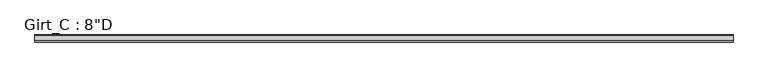
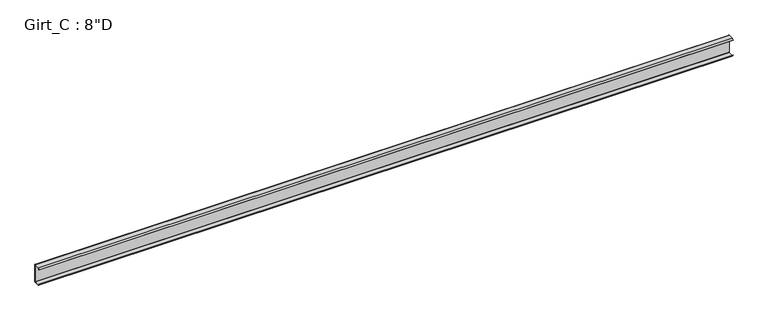
"""IFC4 building model written with IfcOpenShell, lengths in millimetres: beam geometry."""

from ifc_helpers import new_model, si_unit, point, frame, frame_2d, origin, place, context, project, spatial, polyline, circle_curve, trimmed, segment, composite_curve, outline, extrude, source, transform, mapped, element, save


def beam_9492e7bf(model_context):
    return source(origin(), model_context, "Body", "SweptSolid", [
        extrude(outline(composite_curve([segment(polyline([(-63.5, 101.6), (-3.3734375, 101.6)]), True, "CONTINUOUS"), segment(trimmed(circle_curve(frame_2d((-3.3734375, 96.8375)), 4.7625), [point((-3.3734375, 101.6))], [point((1.3890625, 96.8375))], False, "CARTESIAN"), True, "CONTINUOUS"), segment(polyline([(1.3890625, 96.8375), (1.3890625, -96.8375)]), True, "CONTINUOUS"), segment(trimmed(circle_curve(frame_2d((-3.3734375, -96.8375)), 4.7625), [point((1.3890625, -96.8375))], [point((-3.3734375, -101.6))], False, "CARTESIAN"), True, "CONTINUOUS"), segment(polyline([(-3.3734375, -101.6), (-63.5, -101.6), (-75.745104, -87.0068534), (-73.6169367, -85.221109), (-62.204539, -98.821875), (-3.2694106, -98.821875)]), True, "CONTINUOUS"), segment(trimmed(circle_curve(frame_2d((-3.3748024, -96.8389339)), 1.9857399), [point((-3.2694106, -98.821875))], [point((-1.3890625, -96.8389339))], True, "CARTESIAN"), True, "CONTINUOUS"), segment(polyline([(-1.3890625, -96.8389339), (-1.3890625, 96.8381931)]), True, "CONTINUOUS"), segment(trimmed(circle_curve(frame_2d((-3.3741066, 96.8381931)), 1.9850441), [point((-1.3890625, 96.8381931))], [point((-3.3005807, 98.821875))], True, "CARTESIAN"), True, "CONTINUOUS"), segment(polyline([(-3.3005807, 98.821875), (-62.204539, 98.821875), (-73.6169367, 85.221109), (-75.745104, 87.0068534), (-63.5, 101.6)]), True, "CONTINUOUS")], self_intersect=False)), frame((-3690.14375, 0.0, 0.0), z_axis=(1.0, 0.0, 0.0), x_axis=(0.0, 1.0, 0.0)), (0.0, 0.0, 1.0), 7540.625),
    ])


if __name__ == "__main__":
    model = new_model("IFC4")
    model_context = context("Model", 3, world=origin())
    ifc_project = project(units=[si_unit("LENGTHUNIT", "METRE", prefix="MILLI")], contexts=[model_context])
    site = spatial("IfcSite", under=ifc_project)
    building = spatial("IfcBuilding", under=site)
    placement = place(None, origin())
    beam_shape = beam_9492e7bf(model_context)
    element("IfcBeam", 1, ObjectType="Girt_C : 8\"D", at=placement, inside=building, context=model_context, shape_type="MappedRepresentation", body=[
        mapped(beam_shape, transform((0.0, 0.0, 0.0), x_axis=(1.0, 0.0, 0.0), y_axis=(0.0, 1.0, 0.0), z_axis=(0.0, 0.0, 1.0))),
    ])
    save(model, "model.ifc")

# Revit data of these elements
# Type "Girt_C : 8\"D"
#   Web_Thickness = 0' - 0 7/64"
#   Length [instance default] = 10' - 0"
#   Leg_1 = 0' - 2 1/2"
#   Height = 0' - 8"
#   Structural Material [instance default] = none
# Element 1 (IfcBeam, "Girt_C : 8\"D")
#   Structural Material = Steel
#   Materials on its faces: "Steel"
# Materials
#   "Steel": class "Metal", colour RGB 118 118 114, transparency 0, Description = "Steel, mill finish", Cost = 0
